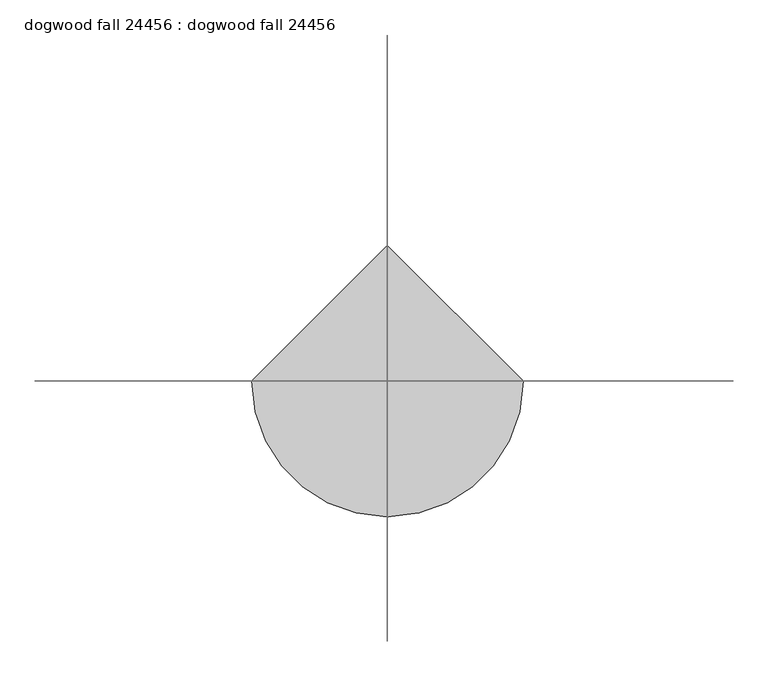
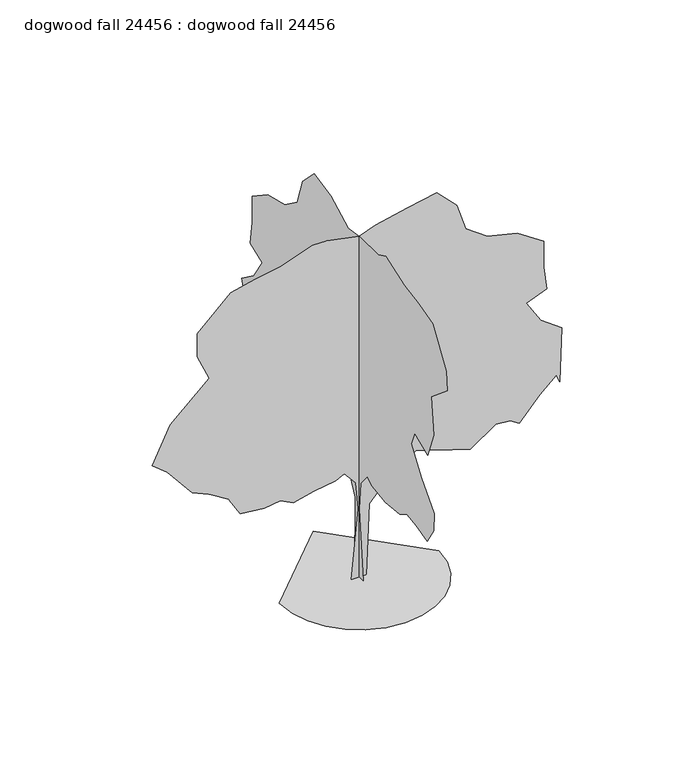
"""IFC4 building model written with IfcOpenShell, lengths in millimetres: proxy geometry, dogwood fall 24456 : dogwood fall 24456."""

from ifc_helpers import new_model, si_unit, origin, place, context, project, spatial, triangles, source, transform, mapped, element, save


def dogwood_fall_24456_dogwood_fall_24456_6d0aa78f(model_context):
    return source(origin(), model_context, "Body", "Tessellation", [
        triangles([(-192.3109178, 0.0008205, 1.6e-05), (-16.7271074, 0.000604, 1752.3067039), (-82.409859, 0.0005256, 2433.5302391), (-353.0958529, 0.0004982, 2763.242672), (-569.1154072, 0.0005207, 2653.3368805), (-1096.3715235, 0.0005536, 2570.9901627), (-1591.7608349, 0.0005886, 2458.5365616), (-1898.5905075, 0.0005841, 2609.3695061), (-2290.9167057, 0.0006068, 2562.43022), (-2869.8722099, 0.0006257, 2615.7702782), (-3136.7753952, 0.000585, 3055.3684456), (-3152.4726929, 0.0005333, 3494.966613), (-3708.9616905, 0.0005642, 3439.7470184), (-4023.1599541, 0.0005631, 3563.9530998), (-4628.8744354, 0.0005018, 4300.1726967), (-4991.8406525, 0.0004841, 4581.9351494), (-4556.966906, 0.0003575, 5484.6012726), (-3614.956382, 0.000214, 6343.3250198), (-3911.1458611, 0.0001503, 6985.7422028), (-3903.2972122, 7.94e-05, 7577.76595), (-3096.8467278, -4.63e-05, 8336.7946198), (-2500.2383766, -8.93e-05, 8478.0947159), (-1903.6324963, -0.0001284, 8588.000798), (-1118.6219822, -0.0001946, 8854.904274), (-771.39354, -0.0002089, 8847.665181), (-0.869176, -0.0002211, 8688.9149872), (388.597465, -0.0002589, 8842.2294662), (1173.6053993, -0.0003135, 9011.9016678), (1870.3457199, -0.0003597, 9144.0075577), (2351.1223331, -0.0003238, 8666.5122849), (2570.9137138, -0.0002529, 7991.4052368), (3089.0233681, -0.0002306, 7614.5956787), (3811.2475983, -0.0002416, 7441.9009872), (4454.9350525, -0.000218, 7007.9420105), (4454.9350525, -0.0001387, 6342.8674896), (4533.4465393, -7.29e-05, 5761.9692261), (4031.0338921, -2.85e-05, 5573.5772369), (4388.5646851, 2.18e-05, 5020.4662308), (4894.5587997, 4.42e-05, 4647.2640106), (4848.1526207, 0.000208, 3289.937558), (4753.969416, 0.0001897, 3478.3295471), (4360.7515572, 0.0002491, 3124.3296432), (3866.7974052, 0.0003366, 2571.3456642), (3646.9858223, 0.0003293, 2712.646051), (3294.3573463, 0.0003402, 2750.8730782), (2682.9278069, 0.000418, 2322.1969185), (2243.6473526, 0.0004213, 2455.8059143), (1819.7412506, 0.0004211, 2612.7983665), (1364.0674656, 0.0004254, 2744.2944099), (1052.0104231, 0.0004704, 2480.6293991), (671.2006004, 0.0005133, 2260.8278446), (558.848701, 0.0005335, 2132.7584816), (248.3812054, 0.0005887, 1782.9289627), (173.4511497, 0.0008045, 0.0), (0.0021376, -182.7973452, 0.0005248), (0.0021882, -7.2139106, 1752.3067039), (0.0022151, -72.8967905, 2433.5302391), (0.002184, -343.5835339, 2763.242672), (0.0021697, -559.6030881, 2653.3368805), (0.0021094, -1086.8566973, 2570.9901627), (0.0020516, -1705.7155071, 2637.6395828), (0.0020124, -2004.0209908, 2810.334565), (0.0019932, -2396.3471889, 2763.4205681), (0.0019341, -2851.8381363, 2637.6651627), (0.0019079, -3118.7416122, 3077.2377502), (0.0019265, -3134.4386192, 3516.8359177), (0.0020103, -2600.631958, 4129.1543564), (0.0020549, -2179.9109814, 4728.6709602), (0.0020635, -2333.7258659, 5080.359668), (0.0019965, -2867.535434, 4851.3530067), (0.0019806, -3118.7416122, 5510.7630478), (0.0020252, -3024.5328278, 6437.0762741), (0.0019867, -3683.9428688, 6986.5805237), (0.0020094, -3636.8509758, 7457.5982849), (0.0020718, -3087.3217278, 8336.7946198), (0.0021378, -2490.7258759, 8478.0947159), (0.0022024, -1894.1201408, 8588.000798), (0.0023157, -1109.1096994, 8854.904274), (0.0023226, -810.8067593, 8713.6041779), (0.0024229, -41.4965223, 8697.9574585), (0.0024414, 460.9087852, 8619.3953934), (0.0025575, 1183.1176821, 9011.9016678), (0.0026275, 1879.8580753, 9144.0075577), (0.0026613, 2360.6346886, 8666.5122849), (0.0026751, 2580.4390045, 7991.4052368), (0.0027149, 3098.5483681, 7614.5956787), (0.0027726, 3820.7473091, 7441.9009872), (0.0028155, 4464.4600525, 7007.9420105), (0.0028201, 4464.4600525, 6342.8674896), (0.0027982, 4542.9715393, 5761.9692261), (0.0027343, 4040.5588921, 5573.5772369), (0.0027594, 4398.0643959, 5020.4662308), (0.0027989, 4904.0582199, 4647.2640106), (0.0027392, 4542.9715393, 3642.4390068), (0.0027433, 4448.7627548, 3830.8565758), (0.0026849, 4009.1645874, 3705.2534866), (0.0026458, 3726.5385246, 3092.9350479), (0.0026087, 3506.7522308, 3234.2354347), (0.0025162, 2622.0948921, 3545.5126556), (0.0025005, 2219.0194954, 3587.3464394), (0.0024795, 2172.2325256, 3155.7492371), (0.0024342, 1748.326569, 3312.7469215), (0.0023792, 1293.0210754, 3281.3523262), (0.0023341, 1061.5252493, 2480.6293991), (0.0022742, 680.7129559, 2260.8278446), (0.0022755, 445.2090168, 2527.7311752), (0.0022371, 161.7295541, 1931.4277473), (0.0021873, 182.964468, 2.94e-05), (-1921.704649, 0.0, 0.008716), (-1870.8994652, -440.32712, 0.0086613), (-1726.2133839, -844.6980045, 0.0086067), (-1499.2260761, -1201.5251341, 0.0085542), (-1201.5251341, -1499.2260761, 0.0085058), (-844.6980045, -1726.2107677, 0.0084631), (-440.32712, -1870.8994652, 0.0084282), (7.39e-05, -1921.704649, 0.0084029), (440.32712, -1870.8994652, 0.0083897), (844.6980045, -1726.2133839, 0.0083892), (1201.5251341, -1499.2260761, 0.0084007), (1499.2260761, -1201.5251341, 0.0084232), (1726.2133839, -844.6980045, 0.0084558), (1870.8994652, -440.32712, 0.0084977), (1921.704649, 0.000168, 0.0085479), (-0.0002634, 1921.704649, 0.0088611)], [[39, 40, 41], [46, 47, 48], [42, 43, 44], [54, 1, 2], [53, 54, 2], [53, 2, 3], [52, 53, 3], [15, 16, 17], [38, 39, 41], [50, 51, 52], [49, 50, 52], [35, 36, 37], [38, 41, 42], [9, 10, 11], [15, 17, 18], [9, 11, 12], [9, 12, 13], [8, 9, 13], [42, 44, 45], [38, 42, 45], [37, 38, 45], [37, 45, 46], [52, 3, 4], [8, 13, 14], [49, 52, 4], [33, 34, 35], [33, 35, 37], [32, 33, 37], [32, 37, 46], [31, 32, 46], [18, 19, 20], [18, 20, 21], [18, 21, 22], [18, 22, 23], [28, 29, 30], [28, 30, 31], [27, 28, 31], [27, 31, 46], [26, 27, 46], [26, 46, 48], [26, 48, 49], [26, 49, 4], [25, 26, 4], [25, 4, 5], [25, 5, 6], [25, 6, 7], [25, 7, 8], [25, 8, 14], [25, 14, 15], [25, 15, 18], [25, 18, 23], [25, 23, 24], [93, 94, 95], [100, 101, 102], [96, 97, 98], [108, 55, 56], [107, 108, 56], [107, 56, 57], [106, 107, 57], [69, 70, 71], [92, 93, 95], [104, 105, 106], [103, 104, 106], [89, 90, 91], [92, 95, 96], [63, 64, 65], [69, 71, 72], [63, 65, 66], [63, 66, 67], [62, 63, 67], [96, 98, 99], [92, 96, 99], [91, 92, 99], [91, 99, 100], [106, 57, 58], [62, 67, 68], [103, 106, 58], [87, 88, 89], [87, 89, 91], [86, 87, 91], [86, 91, 100], [85, 86, 100], [72, 73, 74], [72, 74, 75], [72, 75, 76], [72, 76, 77], [82, 83, 84], [82, 84, 85], [81, 82, 85], [81, 85, 100], [80, 81, 100], [80, 100, 102], [80, 102, 103], [80, 103, 58], [79, 80, 58], [79, 58, 59], [79, 59, 60], [79, 60, 61], [79, 61, 62], [79, 62, 68], [79, 68, 69], [79, 69, 72], [79, 72, 77], [79, 77, 78], [123, 124, 109], [122, 123, 109], [122, 109, 110], [121, 122, 110], [121, 110, 111], [121, 111, 112], [120, 121, 112], [119, 120, 112], [119, 112, 113], [119, 113, 114], [119, 114, 115], [119, 115, 116], [119, 116, 117], [119, 117, 118]], closed=False),
    ])


if __name__ == "__main__":
    model = new_model("IFC4")
    model_context = context("Model", 3, world=origin())
    ifc_project = project(units=[si_unit("LENGTHUNIT", "METRE", prefix="MILLI")], contexts=[model_context])
    site = spatial("IfcSite", under=ifc_project)
    building = spatial("IfcBuilding", under=site)
    placement = place(None, origin())
    dogwood_fall_24456_dogwood_fall_24456_shape = dogwood_fall_24456_dogwood_fall_24456_6d0aa78f(model_context)
    element("IfcBuildingElementProxy", 1, Name="dogwood fall 24456 : dogwood fall 24456", ObjectType="dogwood fall 24456 : dogwood fall 24456", at=placement, inside=building, context=model_context, shape_type="MappedRepresentation", body=[
        mapped(dogwood_fall_24456_dogwood_fall_24456_shape, transform((0.0, 0.0, 0.0), x_axis=(1.0, 0.0, 0.0), y_axis=(0.0, 1.0, 0.0), z_axis=(0.0, 0.0, 1.0))),
    ])
    save(model, "model.ifc")

# Revit data of these elements
# Type "dogwood fall 24456 : dogwood fall 24456"
#   built-in parameter 1005195 = "RPC-16-FUM2-EMXX-U4HL-8000-ST1L-LVER-AU"
#   Height = 0
